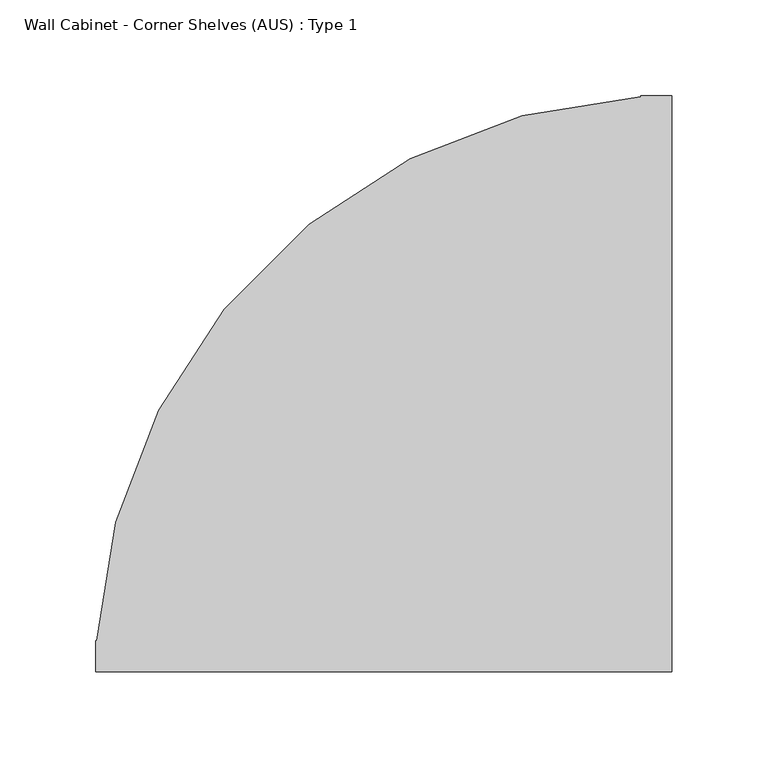
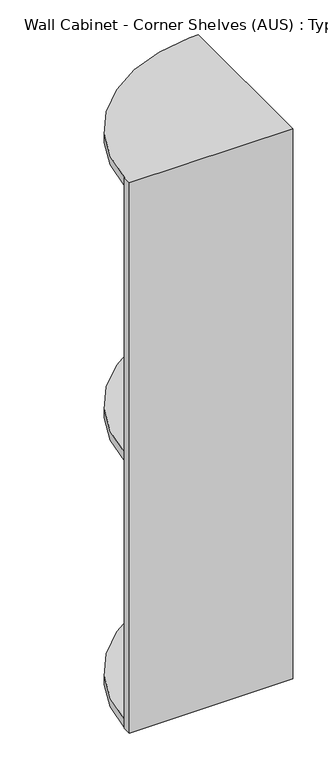
"""IFC4 building model written with IfcOpenShell, lengths in millimetres: furniture geometry, Wall Cabinet - Corner Shelves (AUS) : Type 1."""

from ifc_helpers import new_model, si_unit, frame, origin, place, context, project, spatial, circle_curve, source, transform, mapped, element, save
from ifc_brep_helpers import plane_surface, cylinder_surface, advanced_brep


def wall_cabinet_corner_shelves_aus_type_1_1fef060b(model_context):
    return source(origin(), model_context, "Body", "AdvancedBrep", [
        advanced_brep(
        [(-25.0, 187.6680748, 2566.8), (275.0, 187.6680748, 2566.8), (275.0, 487.6680748, 2566.8), (259.0, 487.6680748, 2566.8), (259.0, 487.2411042, 2566.8), (-24.5730295, 203.6680748, 2566.8), (-25.0, 203.6680748, 2566.8), (-24.5730295, 203.6680748, 2550.8), (259.0, 487.2411042, 2550.8), (259.0, 203.6680748, 2550.8), (-25.0, 187.6680748, 2033.4), (-25.0, 187.6680748, 2017.4), (-25.0, 187.6680748, 1516.0), (-25.0, 187.6680748, 1500.0), (275.0, 187.6680748, 1500.0), (275.0, 187.6680748, 1516.0), (275.0, 187.6680748, 2017.4), (275.0, 187.6680748, 2033.4), (275.0, 487.6680748, 1500.0), (275.0, 487.6680748, 1516.0), (275.0, 487.6680748, 2017.4), (275.0, 487.6680748, 2033.4), (-25.0, 203.6680748, 1500.0), (-24.5730295, 203.6680748, 1500.0), (259.0, 487.2411042, 1500.0), (259.0, 487.6680748, 1500.0), (259.0, 487.2411042, 1516.0), (259.0, 203.6680748, 1516.0), (259.0, 203.6680748, 2017.4), (259.0, 487.2411042, 2017.4), (259.0, 487.2411042, 2033.4), (259.0, 203.6680748, 2033.4), (-24.5730295, 203.6680748, 2033.4), (-24.5730295, 203.6680748, 2017.4), (-24.5730295, 203.6680748, 1516.0)],
        [
            (0, 1),
            (1, 2),
            (2, 3),
            (3, 4),
            (4, 5, circle_curve(frame((275.0, 187.6680748, 2566.8), z_axis=(0.0, 0.0, 1.0), x_axis=(0.0, 1.0, 0.0)), 300.0)),
            (5, 6),
            (6, 0),
            (7, 8, circle_curve(frame((275.0, 187.6680748, 2550.8), z_axis=(0.0, 0.0, -1.0), x_axis=(0.0, 1.0, 0.0)), 300.0)),
            (8, 9),
            (9, 7),
            (0, 10),
            (10, 11),
            (11, 12),
            (12, 13),
            (13, 14),
            (14, 15),
            (15, 16),
            (16, 17),
            (17, 1),
            (14, 18),
            (18, 19),
            (19, 20),
            (20, 21),
            (21, 2),
            (4, 8),
            (7, 5),
            (13, 22),
            (22, 23),
            (23, 24, circle_curve(frame((275.0, 187.6680748, 1500.0), z_axis=(0.0, 0.0, -1.0), x_axis=(0.0, 1.0, 0.0)), 300.0)),
            (24, 25),
            (25, 18),
            (25, 3),
            (24, 26),
            (26, 27),
            (27, 28),
            (28, 29),
            (29, 30),
            (30, 31),
            (31, 9),
            (22, 6),
            (31, 32),
            (32, 33),
            (33, 28),
            (27, 34),
            (34, 23),
            (30, 32, circle_curve(frame((275.0, 187.6680748, 2033.4), z_axis=(0.0, 0.0, 1.0), x_axis=(0.0, 1.0, 0.0)), 300.0)),
            (33, 29, circle_curve(frame((275.0, 187.6680748, 2017.4), z_axis=(0.0, 0.0, -1.0), x_axis=(0.0, 1.0, 0.0)), 300.0)),
            (26, 34, circle_curve(frame((275.0, 187.6680748, 1516.0), z_axis=(0.0, 0.0, 1.0), x_axis=(0.0, 1.0, 0.0)), 300.0)),
        ],
        [
            plane_surface(frame((275.0, 187.6680748, 2566.8), z_axis=(0.0, 0.0, 1.0), x_axis=(1.0, 0.0, 0.0))),
            plane_surface(frame((275.0, 187.6680748, 2550.8), z_axis=(0.0, 0.0, -1.0), x_axis=(-1.0, 0.0, 0.0))),
            plane_surface(frame((-25.0, 187.6680748, 2566.8), z_axis=(0.0, -1.0, 0.0), x_axis=(0.0, 0.0, -1.0))),
            plane_surface(frame((275.0, 187.6680748, 2566.8), z_axis=(1.0, 0.0, 0.0), x_axis=(0.0, 0.0, -1.0))),
            cylinder_surface(frame((275.0, 187.6680748, 2550.8), z_axis=(0.0, 0.0, 1.0), x_axis=(0.0, 1.0, 0.0)), 300.0),
            plane_surface(frame((259.0, 487.6680748, 1500.0), z_axis=(0.0, 0.0, -1.0), x_axis=(1.0, 0.0, 0.0))),
            plane_surface(frame((275.0, 487.6680748, 2566.8), z_axis=(0.0, 1.0, 0.0), x_axis=(0.0, 0.0, -1.0))),
            plane_surface(frame((259.0, 487.6680748, 2566.8), z_axis=(-1.0, 0.0, 0.0), x_axis=(0.0, 0.0, -1.0))),
            plane_surface(frame((259.0, 203.6680748, 2566.8), z_axis=(0.0, 1.0, 0.0), x_axis=(0.0, 0.0, -1.0))),
            plane_surface(frame((-25.0, 203.6680748, 2566.8), z_axis=(-1.0, 0.0, 0.0), x_axis=(0.0, 0.0, -1.0))),
            plane_surface(frame((275.0, 187.6680748, 2033.4), z_axis=(0.0, 0.0, 1.0), x_axis=(1.0, 0.0, 0.0))),
            plane_surface(frame((275.0, 187.6680748, 2017.4), z_axis=(0.0, 0.0, -1.0), x_axis=(-1.0, 0.0, 0.0))),
            cylinder_surface(frame((275.0, 187.6680748, 2017.4), z_axis=(0.0, 0.0, 1.0), x_axis=(0.0, 1.0, 0.0)), 300.0),
            plane_surface(frame((275.0, 187.6680748, 1516.0), z_axis=(0.0, 0.0, 1.0), x_axis=(1.0, 0.0, 0.0))),
            cylinder_surface(frame((275.0, 187.6680748, 1500.0), z_axis=(0.0, 0.0, 1.0), x_axis=(0.0, 1.0, 0.0)), 300.0),
        ],
        [
            (0, [[1, 2, 3, 4, 5, 6, 7]]),
            (1, [[8, 9, 10]]),
            (2, [[-1, 11, 12, 13, 14, 15, 16, 17, 18, 19]]),
            (3, [[-2, -19, -18, -17, -16, 20, 21, 22, 23, 24]]),
            (4, [[-5, 25, -8, 26]]),
            (5, [[-20, -15, 27, 28, 29, 30, 31]]),
            (6, [[-3, -24, -23, -22, -21, -31, 32]]),
            (7, [[-32, -30, 33, 34, 35, 36, 37, 38, 39, -9, -25, -4]]),
            (8, [[40, -6, -26, -10, -39, 41, 42, 43, -35, 44, 45, -28]]),
            (9, [[-7, -40, -27, -14, -13, -12, -11]]),
            (10, [[46, -41, -38]]),
            (11, [[47, -36, -43]]),
            (12, [[-46, -37, -47, -42]]),
            (13, [[48, -44, -34]]),
            (14, [[-29, -45, -48, -33]]),
        ],
    ),
    ])


if __name__ == "__main__":
    model = new_model("IFC4")
    model_context = context("Model", 3, world=origin())
    ifc_project = project(units=[si_unit("LENGTHUNIT", "METRE", prefix="MILLI")], contexts=[model_context])
    site = spatial("IfcSite", under=ifc_project)
    building = spatial("IfcBuilding", under=site)
    placement = place(None, origin())
    wall_cabinet_corner_shelves_aus_type_1_shape = wall_cabinet_corner_shelves_aus_type_1_1fef060b(model_context)
    element("IfcFurniture", 1, ObjectType="Wall Cabinet - Corner Shelves (AUS) : Type 1", at=placement, inside=building, context=model_context, shape_type="MappedRepresentation", body=[
        mapped(wall_cabinet_corner_shelves_aus_type_1_shape, transform((0.0, 0.0, 0.0), x_axis=(1.0, 0.0, 0.0), y_axis=(0.0, 1.0, 0.0), z_axis=(0.0, 0.0, 1.0))),
    ])
    save(model, "model.ifc")

# Revit data of these elements
# Type "Wall Cabinet - Corner Shelves (AUS) : Type 1"
#   COBie.Type.CreatedBy = "doug.wood@us.ibm.com"
#   COBie.Type.CreatedOn = "2016-04-14T02:07:23"
#   COBie.Type.Name = "Casework_Wall Cabinet - Corner Shelves (AUS)_Type 1"
#   COBie.Type.Category = "n/a"
#   COBie.Type.Description = "Wall Cabinet - Corner Shelves (AUS)_Type 1"
#   COBie.Type.Manufacturer = ""
#   COBie.Type.ModelNumber = ""
#   COBie.Type.ReplacementCost = 0
#   Width [instance default] = 0' - 11.81102"
#   Height [instance default] = 1' - 11.62205"
#   Depth [instance default] = 0' - 11.81102"
#   COBie.Type = no
#   Show Outline [instance default] = no
#   Show Hidden [instance default] = yes
#   Assembly Code = ""
# Element 1 (IfcFurniture, "Wall Cabinet - Corner Shelves (AUS) : Type 1")
#   Height = 3' - 6"
